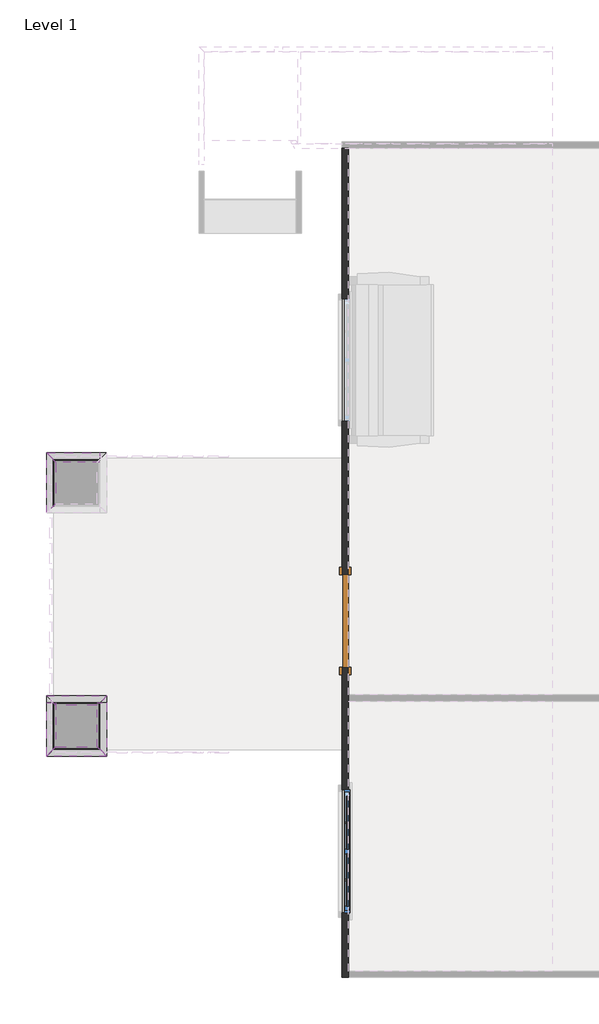
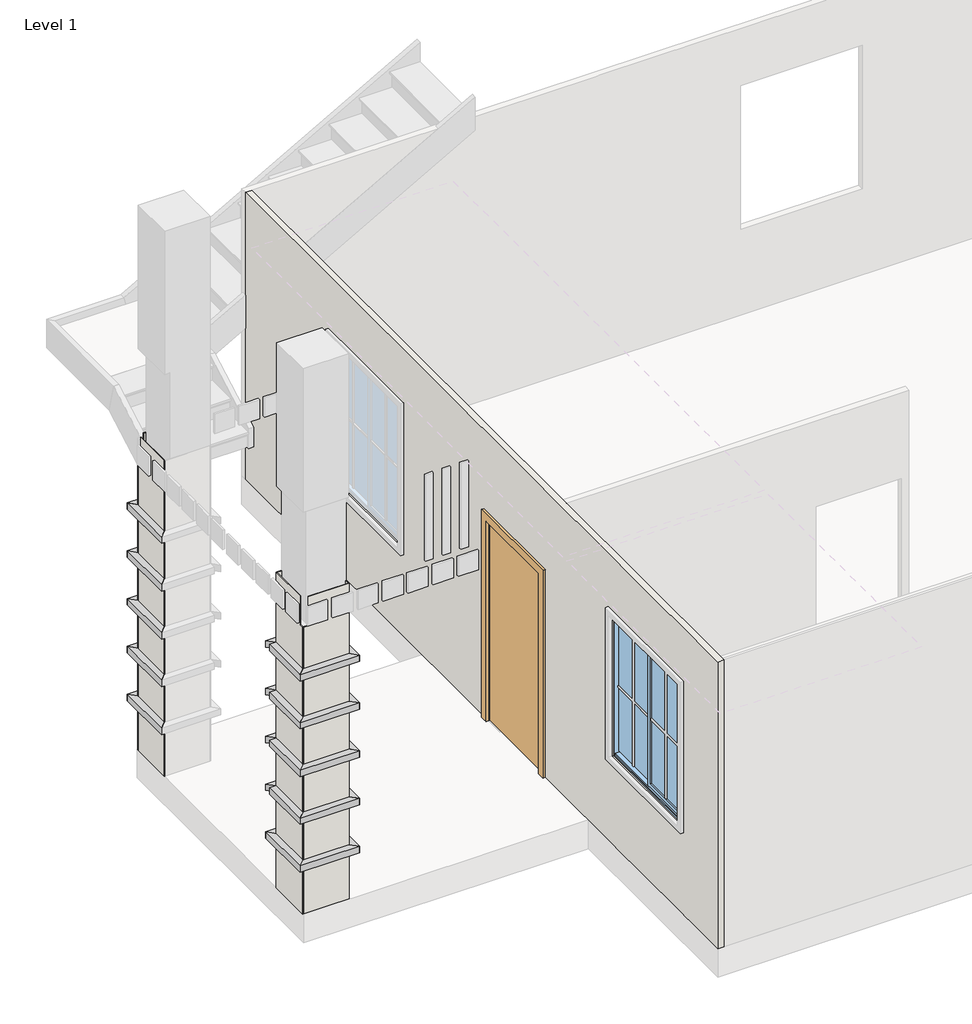
# One storey, part 1 of 3: 31 proxies, 7 walls, 1 door, 1 window.
# Revit data of these elements (continued)
# Type "Single-Flush : 36\" x 84\""
#   Type Mark = "1"
#   Construction Type Id = "MDOOR"
#   Assembly Code = "C1020"
#   Analytic Construction = "Metal"
#   Thickness = 0' - 2"
#   Heat Transfer Coefficient (U) = 0.651978 BTU/(h·ft²·°F)
#   Height = 7' - 0"
#   Trim Projection Ext = 0' - 1"
#   Trim Projection Int = 0' - 1"
#   Trim Width = 0' - 3"
#   Width = 3' - 0"
#   Define Thermal Properties by = 1
#   Define Thermal Properties by = 1
#   Door Material = Door - Panel
#   Frame Material = Door - Frame
#   Visual Light Transmittance = 0
#   Solar Heat Gain Coefficient = 0
#   Function = (empty or 0)
#   Wall Closure = (empty or 0)
# Type "pillarhost"
#   Assembly Code = "B2010"
#   Layers, outside or top first: 0' - 0 1/4" no material (function 1)
# Type "Generic - 8\""
#   Assembly Code = "B2010"
#   Layers, outside or top first: 0' - 2 1/2" no material (function 1)
# Type "Window-Sliding-Double : 48\" x 60\""
#   Type Mark = "19"
#   Fire Rating = "0.5h"
#   Assembly Code = "B2020100"
#   Analytic Construction = "Double glazing - domestic"
#   Window Inset [instance default] = 0' - 0"
#   Wall Thickness [instance default] = 0' - 6"
#   Visual Light Transmittance = 0.81
#   Thermal Resistance (R) = 1.8146 (h·ft²·°F)/BTU
#   Solar Heat Gain Coefficient = 0.76
#   Muntin Width = 1' - 8 5/8"
#   Muntin Height = 4' - 6 1/4"
#   Interior Wall Closure [instance default] = 0' - 2 3/4"
#   Heat Transfer Coefficient (U) = 0.5511 BTU/(h·ft²·°F)
#   Frame Extension [instance default] = 0' - 0 1/4"
#   Exterior Wall Closure [instance default] = 0' - 1 1/4"
#   Rough Width = 4' - 0 1/2"
#   Rough Height = 5' - 0 1/2"
#   Height = 5' - 0"
#   Extension Jamb [instance default] = 0' - 2 3/4"
#   Default Sill Height = 3' - 0"
#   Width = 4' - 0"
#   Interior Trim Visibility [instance default] = yes
#   Indicator Visibility [instance default] = yes
#   Exterior Trim Visibility [instance default] = yes
#   Muntin Visibility = yes
#   Extension Jamb Visibility [instance default] = yes
#   Muntin Pattern = Muntin Pattern_2x2 : Muntin Pattern_2x2
#   Interior Trim Material = Wood - Stained
#   Interior Trim = Trim-Window-Interior-Flat : Picture Frame
#   Interior Frame Material = Wood - Stained
#   Glass Panel Material = Glass
#   Exterior Trim Material = Clad - White
#   Exterior Trim = Trim-Window-Exterior-Flat : with Sill
#   Exterior Frame Material = Clad - White
#   Wall Closure = (empty or 0)
# Element 32 (IfcDoor, "Single-Flush : 36\" x 84\"")
#   Phase Created = New Construction
#   Materials on its faces: "Door - Frame", "Door - Panel"
# Elements 33, 34, 35, 36, 37, 38 (IfcWall, "pillarhost")
#   Top Offset = 0' - 0"
#   Base Offset = 0' - 0"
#   wall height = 11' - 0"
#   Phase Created = New Construction
#   Base Constraint = Level 1
#   Top Constraint = Level 2
#   Materials on its faces: "Default Wall", "Steel, Paint Finish, Ivory, Matte"
# Element 39 (IfcWall, "Generic - 8\"")
#   Top Offset = 0' - 0"
#   Base Offset = 0' - 0"
#   wall height = 10' - 0"
#   Phase Created = New Construction
#   Base Constraint = Level 1
#   Top Constraint = Level 2
#   Materials on its faces: "Default Wall"
# Element 40 (IfcWindow, "Window-Sliding-Double : 48\" x 60\"")
#   Mark = "5"
#   Window Inset = 0' - 0"
#   Interior Wall Closure = 0' - 2 3/4"
#   Frame Extension = 0' - 0 1/4"
#   Exterior Wall Closure = 0' - 1 1/4"
#   Interior Trim Visibility = yes
#   Indicator Visibility = yes
#   Exterior Trim Visibility = yes
#   Phase Created = New Construction
#   Materials on its faces: "Glass", "Wood - Stained", "Clad - White"
# Materials
#   "Door - Panel": class "Wood", colour RGB 210 159 95, transparency 0, Cost = 0
#   "Door - Frame": class "Miscellaneous", colour RGB 118 70 51, transparency 0, Cost = 0
#   "Wood - Stained": class "Wood", colour RGB 224 178 126, transparency 0, Cost = 0
#   "Glass": class "Glass", colour RGB 0 128 192, transparency 0.75, Description = "Soda Lime Glass", Cost = 0
#   "Clad - White": class "Wood", colour RGB 242 242 238, transparency 0, Cost = 0
#   "Default Wall": class "Miscellaneous", colour RGB 128 128 128, transparency 0, Cost = 0
#   "Steel, Paint Finish, Ivory, Matte": class "Metal", colour RGB 247 247 239, transparency 0, Description = "Steel, paint finish, ivory, matte", Cost = 0
# Room at (-6636.192, 7233.828) mm, phase "New Construction", upper level "Level 1", upper offset 10' - 6", lower offset 0' - 0"
#   Number = "1"
#   Name = "Room"
# Room at (-2849.973, 7600.236) mm, phase "New Construction", upper level "Level 1", upper offset 10' - 6", lower offset 0' - 0"
#   Number = "2"
#   Name = "Room"
# Room at (-2849.973, 3162.624) mm, phase "New Construction", upper level "Level 1", upper offset 10' - 0", lower offset 0' - 0"
#   Number = "3"
#   Name = "Room"
# Room at (-6636.192, 3162.624) mm, phase "New Construction", upper level "Level 1", upper offset 10' - 0", lower offset 0' - 0"
#   Number = "4"
#   Name = "Room"
